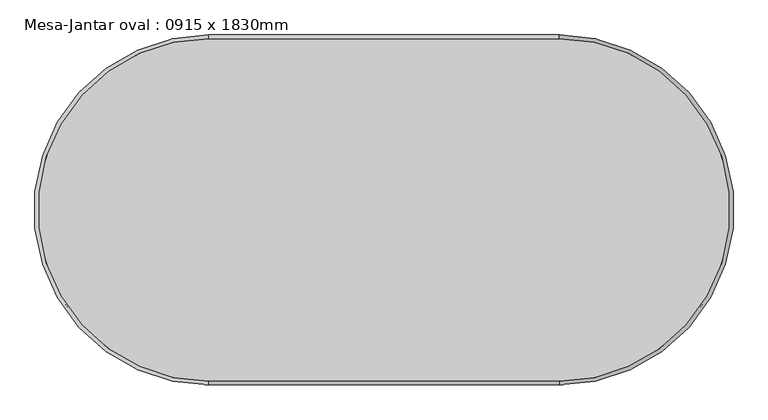
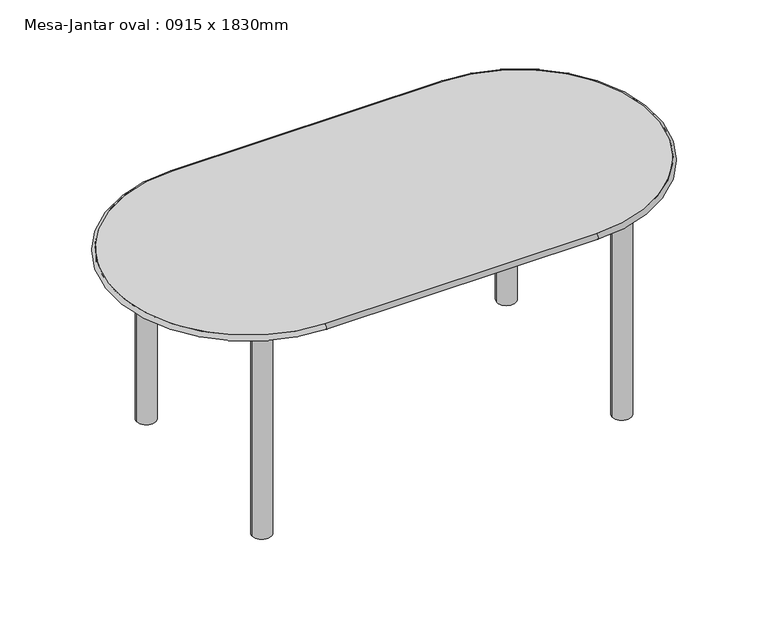
"""IFC4 building model written with IfcOpenShell, lengths in millimetres: furniture geometry, Mesa-Jantar oval : 0915 x 1830mm."""

from ifc_helpers import new_model, si_unit, point, frame, frame_2d, origin, origin_with_axes, place, context, project, spatial, polyline, circle_curve, ellipse_curve, trimmed, segment, composite_curve, outline, extrude, source, transform, mapped, element, save
from ifc_brep_helpers import plane_surface, cylinder_surface, revolved_surface, advanced_brep


def mesa_jantar_oval_0915_x_1830mm_a7cfbe21(model_context):
    return source(origin(), model_context, "Body", "SolidModel", [
        advanced_brep(
        [(-859.3196721, -806.0733607, 762.0), (-859.3196721, -806.0733607, 742.95), (55.6803279, -806.0733607, 742.95), (55.6803279, -806.0733607, 762.0), (55.6803279, 89.8766393, 762.0), (55.6803279, 89.8766393, 742.95), (-859.3196721, 89.8766393, 742.95), (-859.3196721, 89.8766393, 762.0)],
        [
            (0, 1, circle_curve(frame((-859.3196721, -806.0733607, 752.475), z_axis=(1.0, 0.0, 0.0), x_axis=(0.0, 1.0, 0.0)), 9.525)),
            (1, 2),
            (2, 3, circle_curve(frame((55.6803279, -806.0733607, 752.475), z_axis=(-1.0, 0.0, 0.0), x_axis=(0.0, 1.0, 0.0)), 9.525)),
            (3, 0),
            (1, 0),
            (3, 2),
            (4, 3, circle_curve(frame((55.6803279, -358.0983607, 762.0), z_axis=(0.0, 0.0, -1.0), x_axis=(0.0, -1.0, 0.0)), 447.975)),
            (2, 5, circle_curve(frame((55.6803279, -358.0983607, 742.95), z_axis=(0.0, 0.0, 1.0), x_axis=(0.0, -1.0, 0.0)), 447.975)),
            (5, 4, circle_curve(frame((55.6803279, 89.8766393, 752.475), z_axis=(1.0, 0.0, 0.0), x_axis=(0.0, -1.0, 0.0)), 9.525)),
            (4, 5),
            (5, 6),
            (6, 7, circle_curve(frame((-859.3196721, 89.8766393, 752.475), z_axis=(1.0, 0.0, 0.0), x_axis=(0.0, -1.0, 0.0)), 9.525)),
            (7, 4),
            (7, 6),
            (0, 7, circle_curve(frame((-859.3196721, -358.0983607, 762.0), z_axis=(0.0, 0.0, -1.0), x_axis=(0.0, 1.0, 0.0)), 447.975)),
            (6, 1, circle_curve(frame((-859.3196721, -358.0983607, 742.95), z_axis=(0.0, 0.0, 1.0), x_axis=(0.0, 1.0, 0.0)), 447.975)),
        ],
        [
            cylinder_surface(frame((-859.3196721, -806.0733607, 752.475), z_axis=(-1.0, 0.0, 0.0), x_axis=(0.0, 1.0, 0.0)), 9.525),
            plane_surface(frame((-859.3196721, -806.0733607, 762.0), z_axis=(0.0, 1.0, 0.0), x_axis=(1.0, 0.0, 0.0))),
            revolved_surface(trimmed(ellipse_curve(frame((55.6803279, -806.0733607, 752.475), z_axis=(-1.0, 0.0, 0.0), x_axis=(0.0, 1.0, 0.0)), 9.525, 9.525), [point((55.6803279, -806.0733607, 742.95))], [point((55.6803279, -806.0733607, 762.0))], True, "CARTESIAN"), (55.6803279, -358.0983607, 0.0), (0.0, 0.0, 1.0)),
            revolved_surface(polyline([(55.6803279, -806.0733607, 762.0), (55.6803279, -806.0733607, 742.95)]), (55.6803279, -358.0983607, 0.0), (0.0, 0.0, 1.0)),
            cylinder_surface(frame((55.6803279, 89.8766393, 752.475), z_axis=(1.0, 0.0, 0.0), x_axis=(0.0, -1.0, 0.0)), 9.525),
            plane_surface(frame((55.6803279, 89.8766393, 762.0), z_axis=(0.0, -1.0, 0.0), x_axis=(-1.0, 0.0, 0.0))),
            revolved_surface(trimmed(ellipse_curve(frame((-859.3196721, 89.8766393, 752.475), z_axis=(1.0, 0.0, 0.0), x_axis=(0.0, -1.0, 0.0)), 9.525, 9.525), [point((-859.3196721, 89.8766393, 742.95))], [point((-859.3196721, 89.8766393, 762.0))], True, "CARTESIAN"), (-859.3196721, -358.0983607, 0.0), (0.0, 0.0, 1.0)),
            revolved_surface(polyline([(-859.3196721, 89.87663930000002, 762.0), (-859.3196721, 89.87663930000002, 742.95)]), (-859.3196721, -358.0983607, 0.0), (0.0, 0.0, 1.0)),
        ],
        [
            (0, [[1, 2, 3, 4]]),
            (1, [[5, -4, 6, -2]]),
            (2, [[7, -3, 8, 9]]),
            (3, [[-8, -6, -7, 10]]),
            (4, [[-9, 11, 12, 13]]),
            (5, [[-10, -13, 14, -11]]),
            (6, [[15, -12, 16, -1]]),
            (7, [[-16, -14, -15, -5]]),
        ],
    ),
        extrude(outline(composite_curve([segment(trimmed(circle_curve(frame_2d((-1008.5446721, -21.2483607)), 31.75), [point((-1040.2946721, -21.2483607))], [point((-976.7946721, -21.2483607))], False, "CARTESIAN"), True, "CONTINUOUS"), segment(trimmed(circle_curve(frame_2d((-1008.5446721, -21.2483607)), 31.75), [point((-976.7946721, -21.2483607))], [point((-1040.2946721, -21.2483607))], False, "CARTESIAN"), True, "CONTINUOUS")], self_intersect=False)), origin_with_axes(), (0.0, 0.0, 1.0), 742.95),
        extrude(outline(composite_curve([segment(trimmed(circle_curve(frame_2d((-1008.5446721, -694.9483607)), 31.75), [point((-1040.2946721, -694.9483607))], [point((-976.7946721, -694.9483607))], False, "CARTESIAN"), True, "CONTINUOUS"), segment(trimmed(circle_curve(frame_2d((-1008.5446721, -694.9483607)), 31.75), [point((-976.7946721, -694.9483607))], [point((-1040.2946721, -694.9483607))], False, "CARTESIAN"), True, "CONTINUOUS")], self_intersect=False)), origin_with_axes(), (0.0, 0.0, 1.0), 742.95),
        extrude(outline(composite_curve([segment(trimmed(circle_curve(frame_2d((204.9053279, -21.2483607)), 31.75), [point((173.1553279, -21.2483607))], [point((236.6553279, -21.2483607))], False, "CARTESIAN"), True, "CONTINUOUS"), segment(trimmed(circle_curve(frame_2d((204.9053279, -21.2483607)), 31.75), [point((236.6553279, -21.2483607))], [point((173.1553279, -21.2483607))], False, "CARTESIAN"), True, "CONTINUOUS")], self_intersect=False)), origin_with_axes(), (0.0, 0.0, 1.0), 742.95),
        extrude(outline(composite_curve([segment(trimmed(circle_curve(frame_2d((204.9053279, -694.9483607)), 31.75), [point((173.1553279, -694.9483607))], [point((236.6553279, -694.9483607))], False, "CARTESIAN"), True, "CONTINUOUS"), segment(trimmed(circle_curve(frame_2d((204.9053279, -694.9483607)), 31.75), [point((236.6553279, -694.9483607))], [point((173.1553279, -694.9483607))], False, "CARTESIAN"), True, "CONTINUOUS")], self_intersect=False)), origin_with_axes(), (0.0, 0.0, 1.0), 742.95),
        extrude(outline(polyline([(223.9553279, -2.1983607), (223.9553279, -713.9983607), (-1027.5946721, -713.9983607), (-1027.5946721, -2.1983607), (223.9553279, -2.1983607)]), holes=[polyline([(204.9053279, -21.2483607), (-1008.5446721, -21.2483607), (-1008.5446721, -694.9483607), (204.9053279, -694.9483607), (204.9053279, -21.2483607)])]), frame((0.0, 0.0, 692.15), z_axis=(0.0, 0.0, 1.0), x_axis=(1.0, 0.0, 0.0)), (0.0, 0.0, 1.0), 50.8),
        extrude(outline(composite_curve([segment(polyline([(-859.3196721, 89.8766393), (55.6803279, 89.8766393)]), True, "CONTINUOUS"), segment(trimmed(circle_curve(frame_2d((55.6803279, -358.0983607)), 447.975), [point((55.6803279, 89.8766393))], [point((503.6553279, -358.0983607))], False, "CARTESIAN"), True, "CONTINUOUS"), segment(trimmed(circle_curve(frame_2d((55.6803279, -358.0983607)), 447.975), [point((503.6553279, -358.0983607))], [point((55.6803279, -806.0733607))], False, "CARTESIAN"), True, "CONTINUOUS"), segment(polyline([(55.6803279, -806.0733607), (-859.3196721, -806.0733607)]), True, "CONTINUOUS"), segment(trimmed(circle_curve(frame_2d((-859.3196721, -358.0983607)), 447.975), [point((-859.3196721, -806.0733607))], [point((-1307.2946721, -358.0983607))], False, "CARTESIAN"), True, "CONTINUOUS"), segment(trimmed(circle_curve(frame_2d((-859.3196721, -358.0983607)), 447.975), [point((-1307.2946721, -358.0983607))], [point((-859.3196721, 89.8766393))], False, "CARTESIAN"), True, "CONTINUOUS")], self_intersect=False)), frame((0.0, 0.0, 742.95), z_axis=(0.0, 0.0, 1.0), x_axis=(1.0, 0.0, 0.0)), (0.0, 0.0, 1.0), 19.05),
    ])


if __name__ == "__main__":
    model = new_model("IFC4")
    model_context = context("Model", 3, world=origin())
    ifc_project = project(units=[si_unit("LENGTHUNIT", "METRE", prefix="MILLI")], contexts=[model_context])
    site = spatial("IfcSite", under=ifc_project)
    building = spatial("IfcBuilding", under=site)
    placement = place(None, origin())
    mesa_jantar_oval_0915_x_1830mm_shape = mesa_jantar_oval_0915_x_1830mm_a7cfbe21(model_context)
    element("IfcFurniture", 1, ObjectType="Mesa-Jantar oval : 0915 x 1830mm", at=placement, inside=building, context=model_context, shape_type="MappedRepresentation", body=[
        mapped(mesa_jantar_oval_0915_x_1830mm_shape, transform((0.0, 0.0, 0.0), x_axis=(1.0, 0.0, 0.0), y_axis=(0.0, 1.0, 0.0), z_axis=(0.0, 0.0, 1.0))),
    ])
    save(model, "model.ifc")

# Revit data of these elements
# Type "Mesa-Jantar oval : 0915 x 1830mm"
#   Comprimento = 1830 mm
#   Largura = 915 mm
#   Material base = none
#   Material superior = none
#   Default Elevation = 0
# Element 1 (IfcFurniture, "Mesa-Jantar oval : 0915 x 1830mm")
#   Materials on its faces: "Vidro - Claro, Cinza"
# Materials
#   "Vidro - Claro, Cinza": class "Vidro", colour RGB 252 255 255, transparency 0.64
